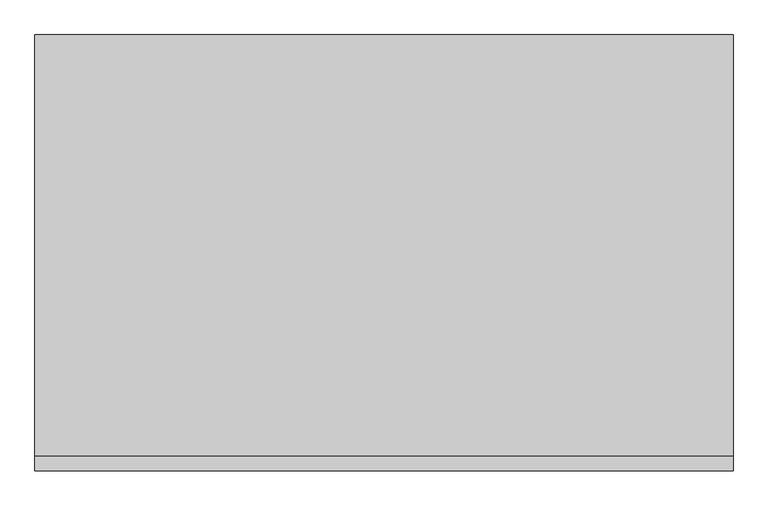
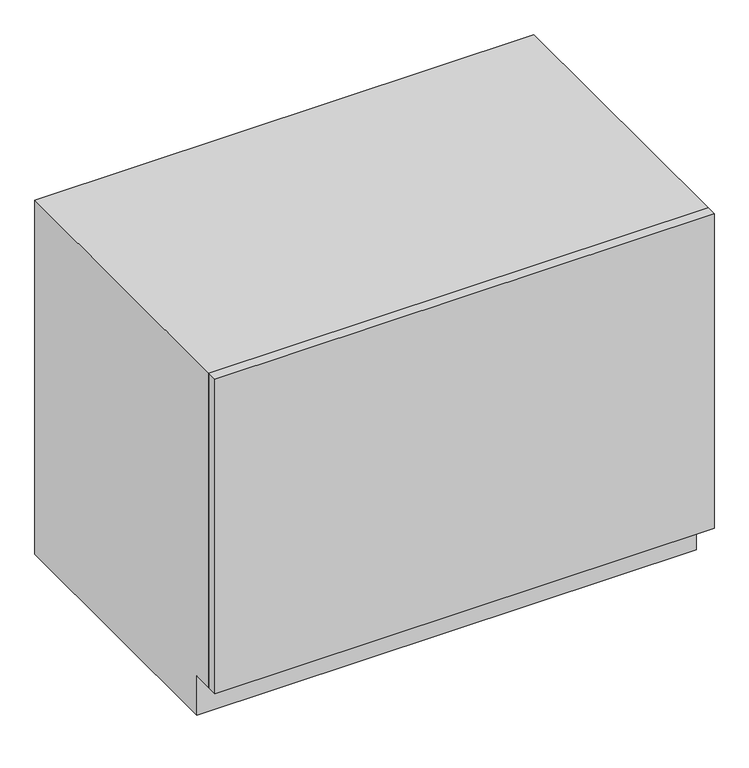
"""IFC4 building model written with IfcOpenShell, lengths in millimetres: furniture geometry, OD_CW_Base Cabinet : OD_CW_Base Cabinet."""

from ifc_helpers import new_model, si_unit, frame, origin, place, context, project, spatial, polyline, outline, extrude, source, transform, mapped, element, save


def furniture_f62fe781(model_context):
    return source(origin(), model_context, "Body", "SweptSolid", [
        extrude(outline(polyline([(18.7377049, -127.0), (1237.9377049, -127.0), (1237.9377049, -152.4), (18.7377049, -152.4), (18.7377049, -127.0)])), frame((0.0, 0.0, 101.6), z_axis=(0.0, 0.0, 1.0), x_axis=(1.0, 0.0, 0.0)), (0.0, 0.0, 1.0), 812.8),
        extrude(outline(polyline([(-127.0, 914.4), (609.6, 914.4), (609.6, 0.0), (-76.2, 0.0), (-76.2, 101.6), (-127.0, 101.6), (-127.0, 914.4)])), frame((18.7377049, 0.0, 0.0), z_axis=(1.0, 0.0, 0.0), x_axis=(0.0, 1.0, 0.0)), (0.0, 0.0, 1.0), 1219.2),
    ])


if __name__ == "__main__":
    model = new_model("IFC4")
    model_context = context("Model", 3, world=origin())
    ifc_project = project(units=[si_unit("LENGTHUNIT", "METRE", prefix="MILLI")], contexts=[model_context])
    site = spatial("IfcSite", under=ifc_project)
    building = spatial("IfcBuilding", under=site)
    placement = place(None, origin())
    furniture_shape = furniture_f62fe781(model_context)
    element("IfcFurniture", 1, ObjectType="OD_CW_Base Cabinet : OD_CW_Base Cabinet", at=placement, inside=building, context=model_context, shape_type="MappedRepresentation", body=[
        mapped(furniture_shape, transform((0.0, 0.0, 0.0), x_axis=(1.0, 0.0, 0.0), y_axis=(0.0, 1.0, 0.0), z_axis=(0.0, 0.0, 1.0))),
    ])
    save(model, "model.ifc")

# Revit data of these elements
# Type "OD_CW_Base Cabinet : OD_CW_Base Cabinet"
#   OD_CW_Width [instance default] = 2' - 10"
#   OD_CW_Length [instance default] = 8' - 0"
#   OD_CW_Height [instance default] = 2' - 3"
#   Depth = 2' - 0"
#   Height = 3' - 0"
#   Width = 4' - 0"
#   OD_CW_Material_Front Panel [instance default] = none
#   OD_CW_Material_Body [instance default] = none
# Element 1 (IfcFurniture, "OD_CW_Base Cabinet : OD_CW_Base Cabinet")
#   OD_CW_Width = 2' - 6"
#   OD_CW_Length = 4' - 0"
#   OD_CW_Height = 3' - 0"
#   OD_CW_Material_Body = CLEAN DISH RACK
#   Materials on its faces: "CLEAN DISH RACK", "CASEWORK"
# Materials
#   "CLEAN DISH RACK": class "Generic", colour RGB 187 187 187, transparency 0, Cost = 0
#   "CASEWORK": class "Generic", colour RGB 181 181 181, transparency 0, Cost = 0
